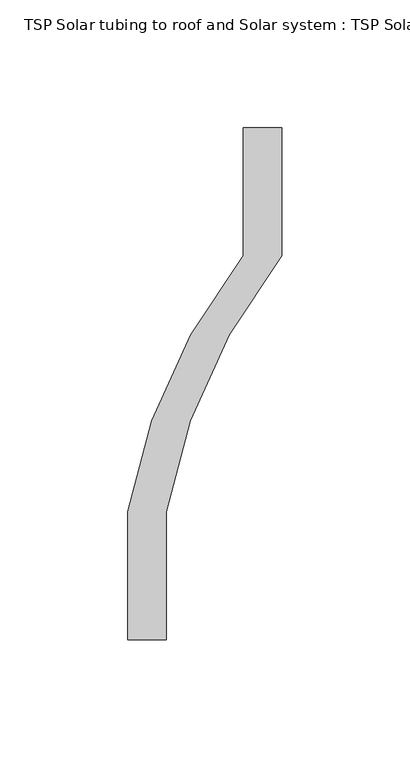
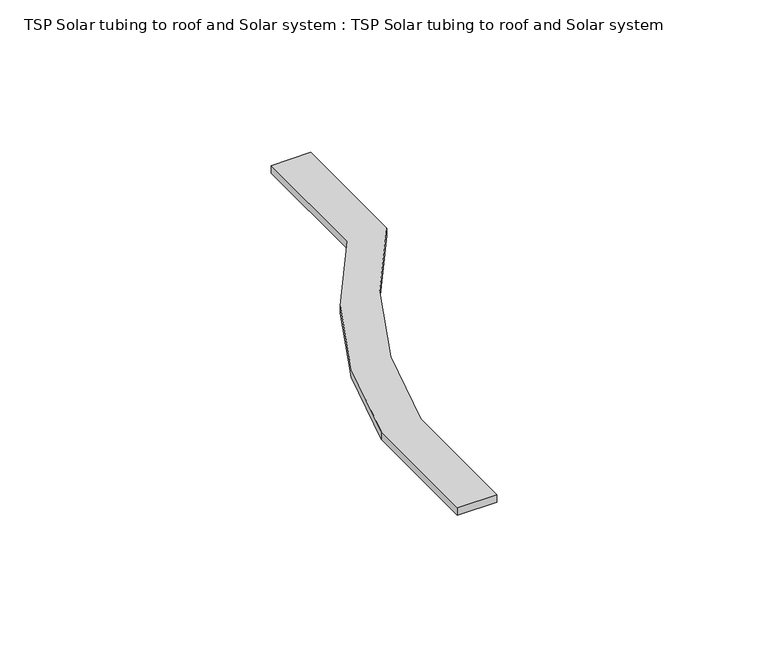
"""IFC4 building model written with IfcOpenShell, lengths in millimetres: proxy geometry, TSP Solar tubing to roof and Solar system : TSP Solar tubing to roof and Solar system."""

from ifc_helpers import new_model, si_unit, point, frame_2d, origin, origin_with_axes, place, context, project, spatial, polyline, circle_curve, trimmed, segment, composite_curve, outline, extrude, source, transform, mapped, element, save


def tsp_solar_tubing_to_roof_and_solar_system_tsp_solar_tubing_5df64f00(model_context):
    return source(origin(), model_context, "Body", "SweptSolid", [
        extrude(outline(composite_curve([segment(polyline([(-26.701468, 100.0), (-11.701468, 100.0), (-11.701468, 50.0)]), True, "CONTINUOUS"), segment(trimmed(circle_curve(frame_2d((162.4439964, -88.490459)), 222.5), [point((-11.701468, 50.0))], [point((-56.701468, -50.0))], True, "CARTESIAN"), True, "CONTINUOUS"), segment(polyline([(-56.701468, -50.0), (-56.701468, -100.0), (-71.701468, -100.0), (-71.701468, -50.0)]), True, "CONTINUOUS"), segment(trimmed(circle_curve(frame_2d((147.4651986, -88.5)), 222.5225332), [point((-71.701468, -50.0))], [point((-26.701468, 50.0))], False, "CARTESIAN"), True, "CONTINUOUS"), segment(polyline([(-26.701468, 50.0), (-26.701468, 100.0)]), True, "CONTINUOUS")], self_intersect=False)), origin_with_axes(), (0.0, 0.0, 1.0), 3.0),
    ])


if __name__ == "__main__":
    model = new_model("IFC4")
    model_context = context("Model", 3, world=origin())
    ifc_project = project(units=[si_unit("LENGTHUNIT", "METRE", prefix="MILLI")], contexts=[model_context])
    site = spatial("IfcSite", under=ifc_project)
    building = spatial("IfcBuilding", under=site)
    placement = place(None, origin())
    tsp_solar_tubing_to_roof_and_solar_system_tsp_solar_tubing_shape = tsp_solar_tubing_to_roof_and_solar_system_tsp_solar_tubing_5df64f00(model_context)
    element("IfcBuildingElementProxy", 1, Name="TSP Solar tubing to roof and Solar system : TSP Solar tubing to roof and Solar system", ObjectType="TSP Solar tubing to roof and Solar system : TSP Solar tubing to roof and Solar system", at=placement, inside=building, context=model_context, shape_type="MappedRepresentation", body=[
        mapped(tsp_solar_tubing_to_roof_and_solar_system_tsp_solar_tubing_shape, transform((0.0, 0.0, 0.0), x_axis=(1.0, 0.0, 0.0), y_axis=(0.0, 1.0, 0.0), z_axis=(0.0, 0.0, 1.0))),
    ])
    save(model, "model.ifc")

# Revit data of these elements
# Type "TSP Solar tubing to roof and Solar system : TSP Solar tubing to roof and Solar system"
#   Model = "TSP_ELECFSTUB"
#   Default Elevation = 0
# Element 1 (IfcBuildingElementProxy, "TSP Solar tubing to roof and Solar system : TSP Solar tubing to roof and Solar system")
#   Materials on its faces: "Plastic, Opaque Black"
# Materials
#   "Plastic, Opaque Black": class "Plastic", colour RGB 0 0 0, transparency 0.7, Description = "Plastic, generic, opaque black", Cost = 0
